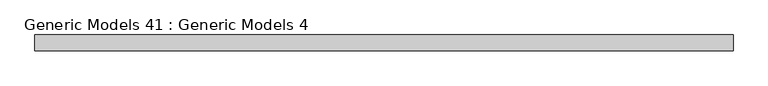
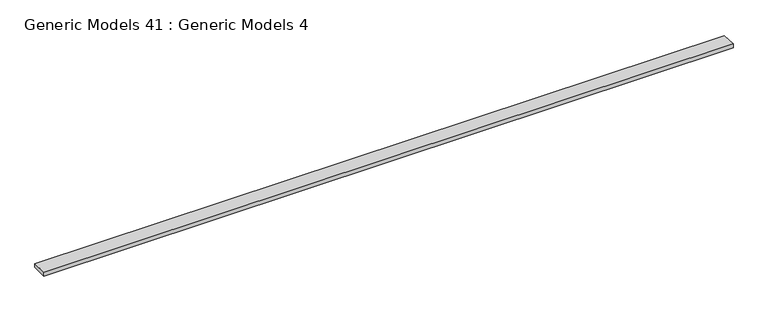
"""IFC4 building model written with IfcOpenShell, lengths in millimetres: proxy geometry, Generic Models 41 : Generic Models 4."""

import ifcopenshell
import ifcopenshell.guid

model = None  # the IFC model being written
_history = None  # IfcOwnerHistory: only IFC2X3 demands one
_inside = {}  # id of a spatial element -> (the spatial element, [elements in it])
_under = {}  # id of a project, library or spatial element -> (it, [spatial elements below it])
_declared = {}  # id of a project -> (the project, [libraries it declares])
_typed = {}  # id of a type object -> (the type object, [elements of that type])
_made_of = {}  # id of a material, layer set ... -> (it, [elements and type objects made of it])


def new_model(schema):
    """Start an empty IFC model of exactly this schema.

    Asked for "IFC4X3", IfcOpenShell would pick the latest addendum, in which some entities
    have other attributes; the version numbers below select the first issue.
    IFC2X3 requires an IfcOwnerHistory on every rooted entity: one is made here for all.
    """
    global model, _history
    if schema == "IFC4X3":
        model = ifcopenshell.file(schema_version=(4, 3, 0, 0))
    else:
        model = ifcopenshell.file(schema=schema)
    _inside.clear()
    _under.clear()
    _declared.clear()
    _typed.clear()
    _made_of.clear()
    _history = None
    if model.schema == "IFC2X3":
        org = make("IfcOrganization", Name="unknown")
        user = make(
            "IfcPersonAndOrganization",
            ThePerson=make("IfcPerson", FamilyName="unknown"),
            TheOrganization=org,
        )
        app = make(
            "IfcApplication",
            ApplicationDeveloper=org,
            Version="unknown",
            ApplicationFullName="unknown",
            ApplicationIdentifier="unknown",
        )
        _history = make(
            "IfcOwnerHistory",
            OwningUser=user,
            OwningApplication=app,
            ChangeAction="ADDED",
            CreationDate=0,
        )
    return model


def make(cls, **values):
    """One entity of the class cls with the attributes given. An attribute that is None is left unset."""
    return model.create_entity(
        cls, **{name: value for name, value in values.items() if value is not None}
    )


def rooted(cls, **values):
    """An entity with a GlobalId (a new one), such as an element, a storey or a relation."""
    return make(cls, GlobalId=ifcopenshell.guid.new(), OwnerHistory=_history, **values)


def si_unit(unit_type, name, prefix=None):
    """IfcSIUnit, for example si_unit("LENGTHUNIT", "METRE", prefix="MILLI")."""
    return make("IfcSIUnit", UnitType=unit_type, Prefix=prefix, Name=name)


def assignment(units):
    """IfcUnitAssignment: the units of a project."""
    return None if units is None else make("IfcUnitAssignment", Units=units)


def point(xyz):
    """IfcCartesianPoint."""
    return None if xyz is None else make("IfcCartesianPoint", Coordinates=xyz)


def direction(xyz):
    """IfcDirection."""
    return None if xyz is None else make("IfcDirection", DirectionRatios=xyz)


def frame(location, z_axis=None, x_axis=None):
    """IfcAxis2Placement3D, a coordinate frame: its origin and axes. An axis left out is left unset."""
    return make(
        "IfcAxis2Placement3D",
        Location=point(location),
        Axis=direction(z_axis),
        RefDirection=direction(x_axis),
    )


def origin():
    """The frame at (0, 0, 0) with its axes left unset."""
    return frame((0.0, 0.0, 0.0))


def place(relative_to, where):
    """IfcLocalPlacement: puts the frame where relative to a parent placement (None: the world)."""
    return make(
        "IfcLocalPlacement", PlacementRelTo=relative_to, RelativePlacement=where
    )


def context(
    kind, dimensions, precision=None, world=None, true_north=None, identifier=None
):
    """IfcGeometricRepresentationContext, for example the 3D "Model" context."""
    return make(
        "IfcGeometricRepresentationContext",
        ContextIdentifier=identifier,
        ContextType=kind,
        CoordinateSpaceDimension=dimensions,
        Precision=precision,
        WorldCoordinateSystem=world,
        TrueNorth=true_north,
    )


def project(units=None, contexts=None):
    """IfcProject with its units and contexts."""
    return rooted(
        "IfcProject",
        Name="project",
        RepresentationContexts=contexts,
        UnitsInContext=assignment(units),
    )


def spatial(cls, under=None, at=None, **own):
    """A site, building, storey or space (cls), placed at a placement, below another one or the project."""
    s = rooted(cls, ObjectPlacement=at, **own)
    if under is not None:
        _under.setdefault(under.id(), (under, []))[1].append(s)
    return s


def polyline(points):
    """IfcPolyline through the points."""
    return make("IfcPolyline", Points=[point(p) for p in points])


def outline(outer, holes=None, kind="AREA"):
    """IfcArbitraryClosedProfileDef: a profile drawn as a closed curve; with holes, ...WithVoids."""
    if holes is None:
        return make("IfcArbitraryClosedProfileDef", ProfileType=kind, OuterCurve=outer)
    return make(
        "IfcArbitraryProfileDefWithVoids",
        ProfileType=kind,
        OuterCurve=outer,
        InnerCurves=holes,
    )


def extrude(swept, where, along, depth):
    """IfcExtrudedAreaSolid: the profile swept, set in the frame where, extruded along a direction by depth."""
    return make(
        "IfcExtrudedAreaSolid",
        SweptArea=swept,
        Position=where,
        ExtrudedDirection=direction(along),
        Depth=depth,
    )


def shape(context_of_items, identifier, shape_type, items):
    """IfcShapeRepresentation: the items that make up one representation, for example the "Body"."""
    return make(
        "IfcShapeRepresentation",
        ContextOfItems=context_of_items,
        RepresentationIdentifier=identifier,
        RepresentationType=shape_type,
        Items=items,
    )


def source(mapping_origin, context_of_items, identifier, shape_type, items):
    """IfcRepresentationMap: a shape defined once, which mapped items show again and again."""
    return make(
        "IfcRepresentationMap",
        MappingOrigin=mapping_origin,
        MappedRepresentation=shape(context_of_items, identifier, shape_type, items),
    )


def transform(
    local_origin,
    x_axis=None,
    y_axis=None,
    z_axis=None,
    scale=None,
    scale2=None,
    scale3=None,
    uniform=True,
):
    """IfcCartesianTransformationOperator3D, or its non-uniform kind. x_axis, y_axis, z_axis: its Axis1, 2, 3."""
    if uniform:
        return make(
            "IfcCartesianTransformationOperator3D",
            Axis1=direction(x_axis),
            Axis2=direction(y_axis),
            LocalOrigin=point(local_origin),
            Scale=scale,
            Axis3=direction(z_axis),
        )
    return make(
        "IfcCartesianTransformationOperator3DnonUniform",
        Axis1=direction(x_axis),
        Axis2=direction(y_axis),
        LocalOrigin=point(local_origin),
        Scale=scale,
        Axis3=direction(z_axis),
        Scale2=scale2,
        Scale3=scale3,
    )


def mapped(mapping_source, mapping_target):
    """IfcMappedItem: shows the shape of a source again, moved by a transform."""
    return make(
        "IfcMappedItem", MappingSource=mapping_source, MappingTarget=mapping_target
    )


def made_of(thing, what):
    """Note that an element or type object is made of a material, layer set ...; save() writes the relation."""
    if what is not None:
        _made_of.setdefault(what.id(), (what, []))[1].append(thing)
    return thing


def element(
    cls,
    number,
    at=None,
    inside=None,
    cuts=None,
    type_object=None,
    material=None,
    context=None,
    identifier="Body",
    shape_type=None,
    held_by="IfcProductDefinitionShape",
    body=None,
    shapes=None,
    **own,
):
    """One element of the class cls, such as IfcWall. Its Tag is "e" and its number.

    at: its placement. inside: the storey or other place that contains it. cuts: it is an
    opening in that element (IfcRelVoidsElement). A single representation is given by context,
    identifier, shape_type and body (its items); several are given by shapes. held_by: the class
    of the entity that holds the representations. save() writes the other relations.
    """
    e = rooted(cls, Tag="e%d" % number, ObjectPlacement=at, **own)
    if body is not None:
        shapes = [shape(context, identifier, shape_type, body)]
    if shapes is not None:
        e.Representation = make(held_by, Representations=shapes)
    if inside is not None:
        _inside.setdefault(inside.id(), (inside, []))[1].append(e)
    if cuts is not None:
        rooted(
            "IfcRelVoidsElement", RelatingBuildingElement=cuts, RelatedOpeningElement=e
        )
    if type_object is not None:
        _typed.setdefault(type_object.id(), (type_object, []))[1].append(e)
    return made_of(e, material)


def aggregate(whole, parts):
    """IfcRelAggregates: a whole, such as a stair, and the parts it consists of."""
    return rooted("IfcRelAggregates", RelatingObject=whole, RelatedObjects=parts)


def save(model, path):
    """Write the relations noted so far, then the file.

    IfcRelAggregates (storeys below a building ...), IfcRelContainedInSpatialStructure (elements
    in a storey), IfcRelDefinesByType, IfcRelAssociatesMaterial and IfcRelDeclares: one each for
    every whole, place, type object, material and project.
    """
    for whole, parts in _under.values():
        aggregate(whole, parts)
    for where, things in _inside.values():
        rooted(
            "IfcRelContainedInSpatialStructure",
            RelatedElements=things,
            RelatingStructure=where,
        )
    for kind, things in _typed.values():
        rooted("IfcRelDefinesByType", RelatedObjects=things, RelatingType=kind)
    for what, things in _made_of.values():
        rooted("IfcRelAssociatesMaterial", RelatedObjects=things, RelatingMaterial=what)
    for by, libraries in _declared.values():
        rooted("IfcRelDeclares", RelatingContext=by, RelatedDefinitions=libraries)
    model.write(path)


def generic_models_41_generic_models_4_a14cedc2(model_context):
    return source(origin(), model_context, "Body", "SweptSolid", [
        extrude(outline(polyline([(14098.1475835, 127104.4735933), (14098.1475835, 127142.5735933), (14237.8475835, 127136.7527599), (14237.8475835, 127104.4735933), (14098.1475835, 127104.4735933)])), frame((-8342.1048025, 0.0, 0.0), z_axis=(1.0, 0.0, 0.0), x_axis=(0.0, 1.0, 0.0)), (0.0, 0.0, 1.0), 6189.931498),
    ])


if __name__ == "__main__":
    model = new_model("IFC4")
    model_context = context("Model", 3, world=origin())
    ifc_project = project(units=[si_unit("LENGTHUNIT", "METRE", prefix="MILLI")], contexts=[model_context])
    site = spatial("IfcSite", under=ifc_project)
    building = spatial("IfcBuilding", under=site)
    placement = place(None, origin())
    generic_models_41_generic_models_4_shape = generic_models_41_generic_models_4_a14cedc2(model_context)
    element("IfcBuildingElementProxy", 1, Name="Generic Models 41 : Generic Models 4", ObjectType="Generic Models 41 : Generic Models 4", at=placement, inside=building, context=model_context, shape_type="MappedRepresentation", body=[
        mapped(generic_models_41_generic_models_4_shape, transform((0.0, 0.0, 0.0), x_axis=(1.0, 0.0, 0.0), y_axis=(0.0, 1.0, 0.0), z_axis=(0.0, 0.0, 1.0))),
    ])
    save(model, "model.ifc")

# Revit data of these elements
# Element 1 (IfcBuildingElementProxy, "Generic Models 41 : Generic Models 4")
#   Materials on its faces: "_2X BLOCKING AS REQUIRED"
# Materials
#   "_2X BLOCKING AS REQUIRED": class "Generic", colour RGB 177 130 114, transparency 0, Cost = 0
